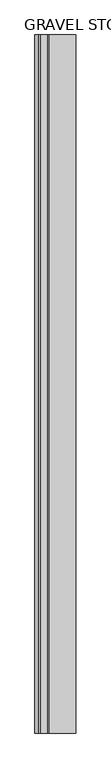
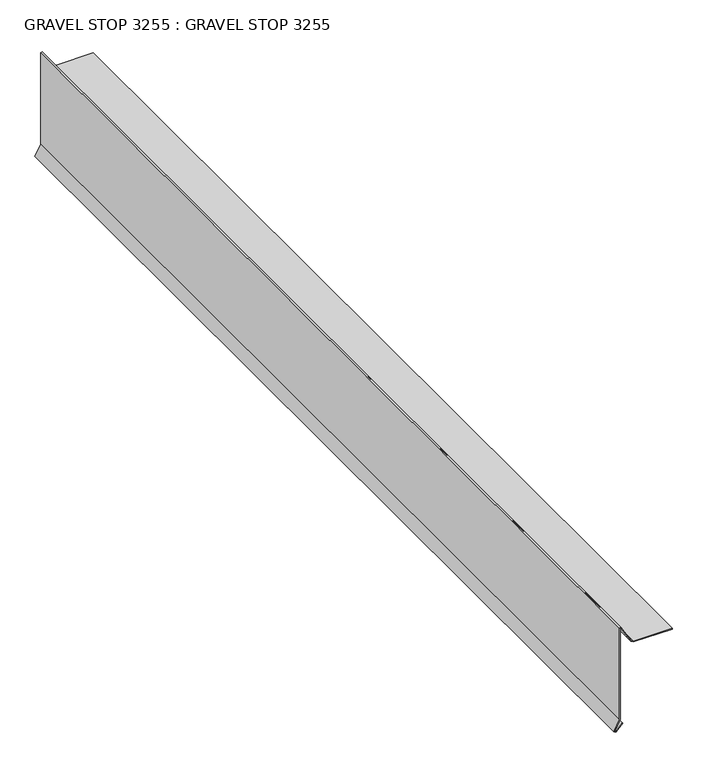
"""IFC4 building model written with IfcOpenShell, lengths in millimetres: proxy geometry, GRAVEL STOP 3255 : GRAVEL STOP 3255."""

from ifc_helpers import new_model, si_unit, frame, origin, place, context, project, spatial, polyline, outline, extrude, source, transform, mapped, element, save


def gravel_stop_3255_gravel_stop_3255_885a835c(model_context):
    return source(origin(), model_context, "Body", "SweptSolid", [
        extrude(outline(polyline([(40077.410403, -2814.9855343), (40091.8049, -2800.5910374), (40092.8027062, -2801.5888435), (40079.2807815, -2815.1107682), (40080.9054201, -2817.2404183), (40101.495749, -2805.9993985), (40293.447969, -2805.9993985), (40293.699878, -2805.0592614), (40258.5078708, -2784.7411466), (40255.9633674, -2780.3339375), (40255.9633674, -2702.4979247), (40257.3744784, -2702.4979247), (40257.3744784, -2779.9558314), (40259.5408757, -2783.7081416), (40295.3431515, -2804.3785952), (40294.5307525, -2807.4105095), (40101.8558531, -2807.4105095), (40080.5182783, -2819.0594785), (40077.410403, -2814.9855343)])), frame((0.0, -1052.8906573, 0.0), z_axis=(0.0, 1.0, 0.0), x_axis=(0.0, 0.0, 1.0)), (0.0, 0.0, 1.0), 2000.25),
    ])


if __name__ == "__main__":
    model = new_model("IFC4")
    model_context = context("Model", 3, world=origin())
    ifc_project = project(units=[si_unit("LENGTHUNIT", "METRE", prefix="MILLI")], contexts=[model_context])
    site = spatial("IfcSite", under=ifc_project)
    building = spatial("IfcBuilding", under=site)
    placement = place(None, origin())
    gravel_stop_3255_gravel_stop_3255_shape = gravel_stop_3255_gravel_stop_3255_885a835c(model_context)
    element("IfcBuildingElementProxy", 1, Name="GRAVEL STOP 3255 : GRAVEL STOP 3255", ObjectType="GRAVEL STOP 3255 : GRAVEL STOP 3255", at=placement, inside=building, context=model_context, shape_type="MappedRepresentation", body=[
        mapped(gravel_stop_3255_gravel_stop_3255_shape, transform((0.0, 0.0, 0.0), x_axis=(1.0, 0.0, 0.0), y_axis=(0.0, 1.0, 0.0), z_axis=(0.0, 0.0, 1.0))),
    ])
    save(model, "model.ifc")

# Revit data of these elements
# Type "GRAVEL STOP 3255 : GRAVEL STOP 3255"
#   NameOverride = "GRAVEL STOP"
# Element 1 (IfcBuildingElementProxy, "GRAVEL STOP 3255 : GRAVEL STOP 3255")
#   Materials on its faces: "GRAVEL STOP REQUIRED WITH GRAVEL SURFACE SYSTEMS"
# Materials
#   "GRAVEL STOP REQUIRED WITH GRAVEL SURFACE SYSTEMS": class "Unassigned", colour RGB 170 170 127, transparency 0
